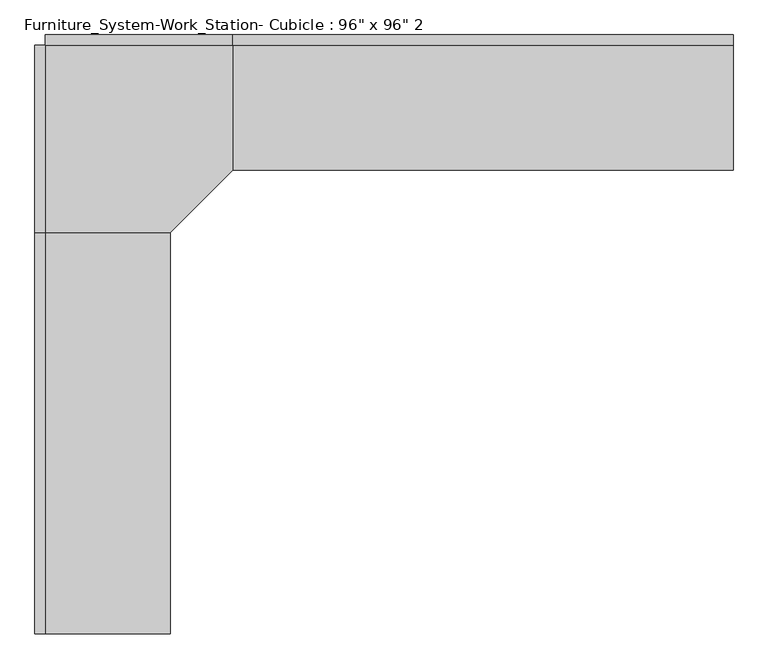
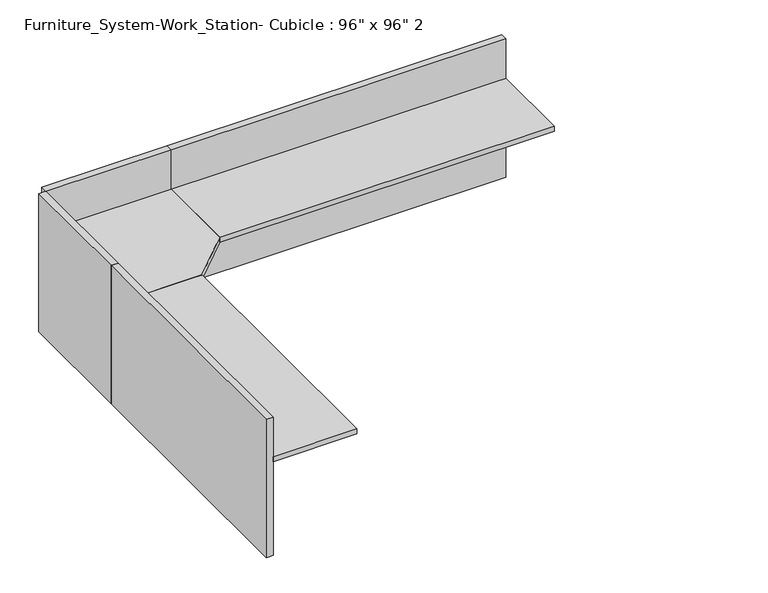
"""IFC4 building model written with IfcOpenShell, lengths in millimetres: furniture geometry."""

from ifc_helpers import new_model, si_unit, frame, origin, origin_with_axes, place, context, project, spatial, polyline, outline, extrude, source, transform, mapped, element, save


def furniture_96e53902(model_context):
    return source(origin(), model_context, "Body", "SweptSolid", [
        extrude(outline(polyline([(-80.9317522, -545.8230076), (833.4682478, -545.8230076), (833.4682478, -1155.4230076), (528.6682478, -1460.2230076), (-80.9317522, -1460.2230076), (-80.9317522, -545.8230076)])), frame((0.0, 0.0, 723.9), z_axis=(0.0, 0.0, 1.0), x_axis=(1.0, 0.0, 0.0)), (0.0, 0.0, 1.0), 38.1),
        extrude(outline(polyline([(528.6682478, -3416.0230076), (-80.9317522, -3416.0230076), (-80.9317522, -1460.2230076), (528.6682478, -1460.2230076), (528.6682478, -3416.0230076)])), frame((0.0, 0.0, 723.9), z_axis=(0.0, 0.0, 1.0), x_axis=(1.0, 0.0, 0.0)), (0.0, 0.0, 1.0), 38.1),
        extrude(outline(polyline([(3271.8682478, -1155.4230076), (833.4682478, -1155.4230076), (833.4682478, -545.8230076), (3271.8682478, -545.8230076), (3271.8682478, -1155.4230076)])), frame((0.0, 0.0, 723.9), z_axis=(0.0, 0.0, 1.0), x_axis=(1.0, 0.0, 0.0)), (0.0, 0.0, 1.0), 38.1),
        extrude(outline(polyline([(3271.8682478, -545.8230076), (833.4682478, -545.8230076), (833.4682478, -495.0230076), (3271.8682478, -495.0230076), (3271.8682478, -545.8230076)])), origin_with_axes(), (0.0, 0.0, 1.0), 1066.8),
        extrude(outline(polyline([(833.4682478, -545.8230076), (-80.9317522, -545.8230076), (-80.9317522, -495.0230076), (833.4682478, -495.0230076), (833.4682478, -545.8230076)])), origin_with_axes(), (0.0, 0.0, 1.0), 1066.8),
        extrude(outline(polyline([(-80.9317522, -1460.2230076), (-131.7317522, -1460.2230076), (-131.7317522, -545.8230076), (-80.9317522, -545.8230076), (-80.9317522, -1460.2230076)])), origin_with_axes(), (0.0, 0.0, 1.0), 1066.8),
        extrude(outline(polyline([(-80.9317522, -3416.0230076), (-131.7317522, -3416.0230076), (-131.7317522, -1460.2230076), (-80.9317522, -1460.2230076), (-80.9317522, -3416.0230076)])), origin_with_axes(), (0.0, 0.0, 1.0), 1066.8),
    ])


if __name__ == "__main__":
    model = new_model("IFC4")
    model_context = context("Model", 3, world=origin())
    ifc_project = project(units=[si_unit("LENGTHUNIT", "METRE", prefix="MILLI")], contexts=[model_context])
    site = spatial("IfcSite", under=ifc_project)
    building = spatial("IfcBuilding", under=site)
    placement = place(None, origin())
    furniture_shape = furniture_96e53902(model_context)
    element("IfcFurniture", 1, ObjectType="Furniture_System-Work_Station- Cubicle : 96\" x 96\" 2", at=placement, inside=building, context=model_context, shape_type="MappedRepresentation", body=[
        mapped(furniture_shape, transform((0.0, 0.0, 0.0), x_axis=(1.0, 0.0, 0.0), y_axis=(0.0, 1.0, 0.0), z_axis=(0.0, 0.0, 1.0))),
    ])
    save(model, "model.ifc")

# Revit data of these elements
# Type "Furniture_System-Work_Station- Cubicle : 96\" x 96\" 2"
#   Assembly Code = "E2020"
#   Desktop Height = 2' - 6"
#   Desktop1 Width = 2' - 0"
#   Desktop2 Width = 2' - 0"
#   Panel Height = 3' - 6"
#   Panel1 Length = 6' - 5"
#   Panel2 Length = 8' - 0"
#   Cube Panel Material = Textile - Light Gray
#   Work Top Material = Laminate - Ivory,Matte
#   Default Elevation = 0
# Element 1 (IfcFurniture, "Furniture_System-Work_Station- Cubicle : 96\" x 96\" 2")
#   Materials on its faces: "Textile - Light Gray", "Laminate - Ivory,Matte"
# Materials
#   "Textile - Light Gray": class "Unassigned", colour RGB 204 204 204, transparency 0
#   "Laminate - Ivory,Matte": class "Unassigned", colour RGB 127 127 127, transparency 0, Comments = "Rendering appearance not upgraded "
